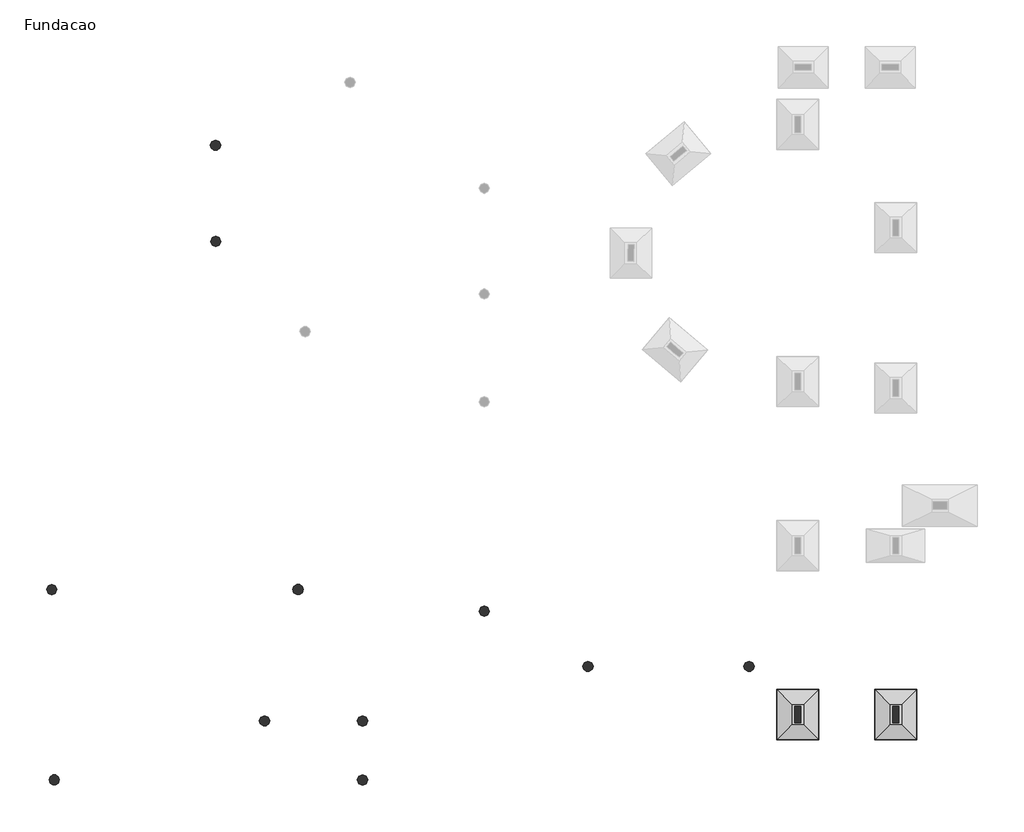
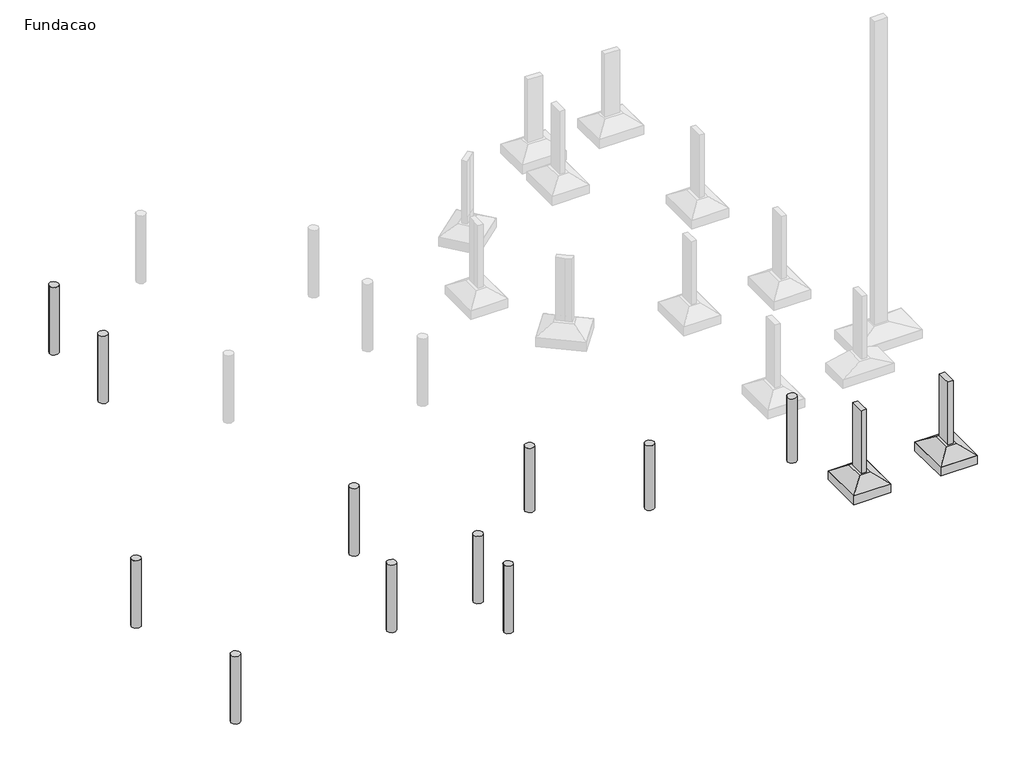
# One storey, part 1 of 2: 13 columns, 2 fasteners.
# Revit data of these elements (continued)
# Element 12 (IfcColumn, "TQS - Pilar retangular : 14.0 x 40.0") (continued)
#   Uso = "ESTRUTURA"
#   Titulo = "PS9"
#   Chave = "PS9//0"
#   Tipo Elemento = "Pilar"
#   SHA1 = "B0C6833D78490A9E7B3F8C386D6833E4B5564321"
#   Revisão = ""
#   Tipo de carga = ""
#   Divisor de flexao = ""
#   Secao = "R 14/40 180°"
#   Configuracao = ""
#   Angulo (graus) = ""
#   Detalhamento = ""
#   Casos de vento manual = ""
#   Tipo = ""
#   Alcas = ""
#   Furos = ""
#   Pino = ""
#   Distribuicao = ""
#   Solidarizado = ""
#   Solidarizar na montagem = ""
#   Unir com o próximo = ""
#   Grupo pre moldado = ""
#   Verificado = ""
#   Concreto C = ""
#   Taxa de armadura (kgf/m³) = 0
#   Carga (tf/m²) = 0
#   Carga (tf/m) = 0
#   Carga (tf) = 0
#   Altura = 1.70 m
#   Rebaixo = 0.00 m
#   Altura da fundacao = 0.00 m
#   Largura = 0.00 m
#   Distancia a face = 0.00 m
#   Distancia ao eixo = 0.00 m
#   Resultado de Ensaios fck (MPa) = 0
#   Unique TQS ID = -966
#   Principal = yes
#   Nasce = yes
#   Morre = yes
#   Cabeca de Pilar = no
#   Structural Material = Concrete - Cast-in-Place Concrete
#   Phase Created = CC_AP/ESTR
#   Materials on its faces: "Concrete - Cast-in-Place Concrete"
# Element 13 (IfcColumn, "TQS - Pilar retangular : 14.0 x 40.0")
#   Uso = "ESTRUTURA"
#   Titulo = "PS10"
#   Chave = "PS10//0"
#   Tipo Elemento = "Pilar"
#   SHA1 = "348E9EB98025B598649ED725E9A09005B776015E"
#   Revisão = ""
#   Tipo de carga = ""
#   Divisor de flexao = ""
#   Secao = "R 14/40 180°"
#   Configuracao = ""
#   Angulo (graus) = ""
#   Detalhamento = ""
#   Casos de vento manual = ""
#   Tipo = ""
#   Alcas = ""
#   Furos = ""
#   Pino = ""
#   Distribuicao = ""
#   Solidarizado = ""
#   Solidarizar na montagem = ""
#   Unir com o próximo = ""
#   Grupo pre moldado = ""
#   Verificado = ""
#   Concreto C = ""
#   Taxa de armadura (kgf/m³) = 0
#   Carga (tf/m²) = 0
#   Carga (tf/m) = 0
#   Carga (tf) = 0
#   Altura = 1.70 m
#   Rebaixo = 0.00 m
#   Altura da fundacao = 0.00 m
#   Largura = 0.00 m
#   Distancia a face = 0.00 m
#   Distancia ao eixo = 0.00 m
#   Resultado de Ensaios fck (MPa) = 0
#   Unique TQS ID = -967
#   Principal = yes
#   Nasce = yes
#   Morre = yes
#   Cabeca de Pilar = no
#   Structural Material = Concrete - Cast-in-Place Concrete
#   Phase Created = CC_AP/ESTR
#   Materials on its faces: "Concrete - Cast-in-Place Concrete"
# Element 14 (IfcFastener, "TQS - Sapata : SPS10")
#   Uso = "ESTRUTURA"
#   Titulo = "SPS10"
#   Chave = "-1543"
#   Tipo Elemento = "Fundação"
#   SHA1 = "612F949682BC8906AE43999ACE3B00A4C616A0A8"
#   Revisão = ""
#   Tipo de carga = ""
#   Divisor de flexao = ""
#   Secao = ""
#   Configuracao = ""
#   Angulo (graus) = ""
#   Detalhamento = ""
#   Casos de vento manual = ""
#   Tipo = "Sapata"
#   Dimensoes = "100.0,120.0"
#   Estacas = ""
#   Calice = ""
#   Rugosidade = ""
#   Alcas = ""
#   Furos = ""
#   Pino = ""
#   Distribuicao = ""
#   Solidarizado = ""
#   Solidarizar na montagem = ""
#   Unir com o próximo = ""
#   Grupo pre moldado = ""
#   Verificado = ""
#   Concreto C = ""
#   Taxa de armadura (kgf/m³) = 0
#   Carga (tf/m²) = 0
#   Carga (tf/m) = 0
#   Carga (tf) = 0
#   Altura = 0.00 m
#   Rebaixo = 0.00 m
#   Pilar ficticio = 0.00 m
#   Topo = -1.45 m
#   Altura total = 0.50 m
#   Rodape = 0.00 m
#   Diametro = 0.00 m
#   Altura dentro do bloco = 0.00 m
#   Entre eixos = 0.00 m
#   Paredes = 0.00 m
#   Caimento = 0.00 m
#   Largura = 0.00 m
#   Distancia a face = 0.00 m
#   Distancia ao eixo = 0.00 m
#   Resultado de Ensaios fck (MPa) = 0
#   Unique TQS ID = -1543
#   Principal = yes
#   Phase Created = CC_AP/ESTR
#   Materials on its faces: "Concreto - Concreto concretado no local"
# Element 15 (IfcFastener, "TQS - Sapata : SPS9")
#   Uso = "ESTRUTURA"
#   Titulo = "SPS9"
#   Chave = "-1542"
#   Tipo Elemento = "Fundação"
#   SHA1 = "96B98524968DB2A66F18ED7D1088E2BB9B4616C7"
#   Revisão = ""
#   Tipo de carga = ""
#   Divisor de flexao = ""
#   Secao = ""
#   Configuracao = ""
#   Angulo (graus) = ""
#   Detalhamento = ""
#   Casos de vento manual = ""
#   Tipo = "Sapata"
#   Dimensoes = "100.0,120.0"
#   Estacas = ""
#   Calice = ""
#   Rugosidade = ""
#   Alcas = ""
#   Furos = ""
#   Pino = ""
#   Distribuicao = ""
#   Solidarizado = ""
#   Solidarizar na montagem = ""
#   Unir com o próximo = ""
#   Grupo pre moldado = ""
#   Verificado = ""
#   Concreto C = ""
#   Taxa de armadura (kgf/m³) = 0
#   Carga (tf/m²) = 0
#   Carga (tf/m) = 0
#   Carga (tf) = 0
#   Altura = 0.00 m
#   Rebaixo = 0.00 m
#   Pilar ficticio = 0.00 m
#   Topo = -1.45 m
#   Altura total = 0.50 m
#   Rodape = 0.00 m
#   Diametro = 0.00 m
#   Altura dentro do bloco = 0.00 m
#   Entre eixos = 0.00 m
#   Paredes = 0.00 m
#   Caimento = 0.00 m
#   Largura = 0.00 m
#   Distancia a face = 0.00 m
#   Distancia ao eixo = 0.00 m
#   Resultado de Ensaios fck (MPa) = 0
#   Unique TQS ID = -1542
#   Principal = yes
#   Phase Created = CC_AP/ESTR
#   Materials on its faces: "Concreto - Concreto concretado no local"
# Materials
#   "Concrete - Cast-in-Place Concrete": class "Unassigned", colour RGB 192 192 192, transparency 0
#   "Concreto - Concreto concretado no local": class "Concreto", colour RGB 192 192 192, transparency 0
